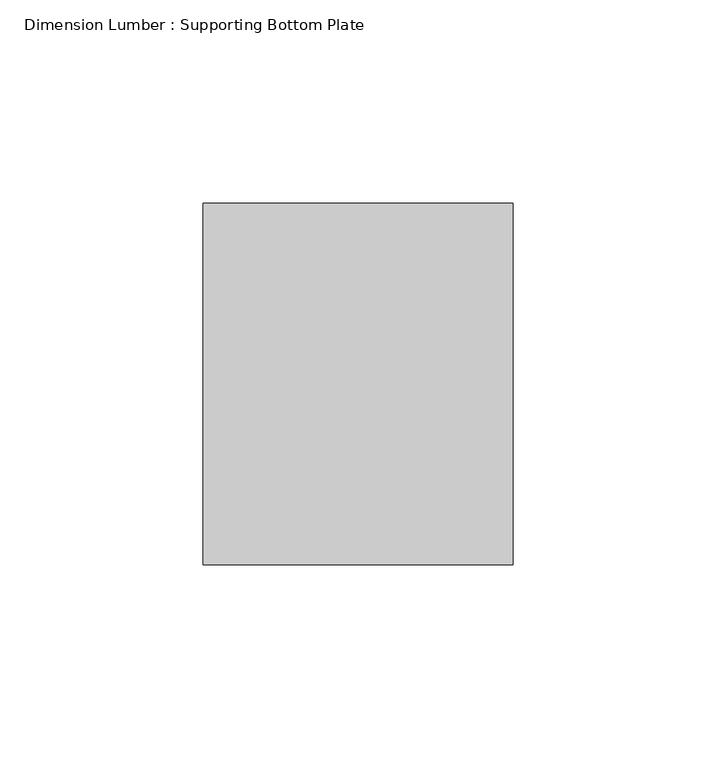
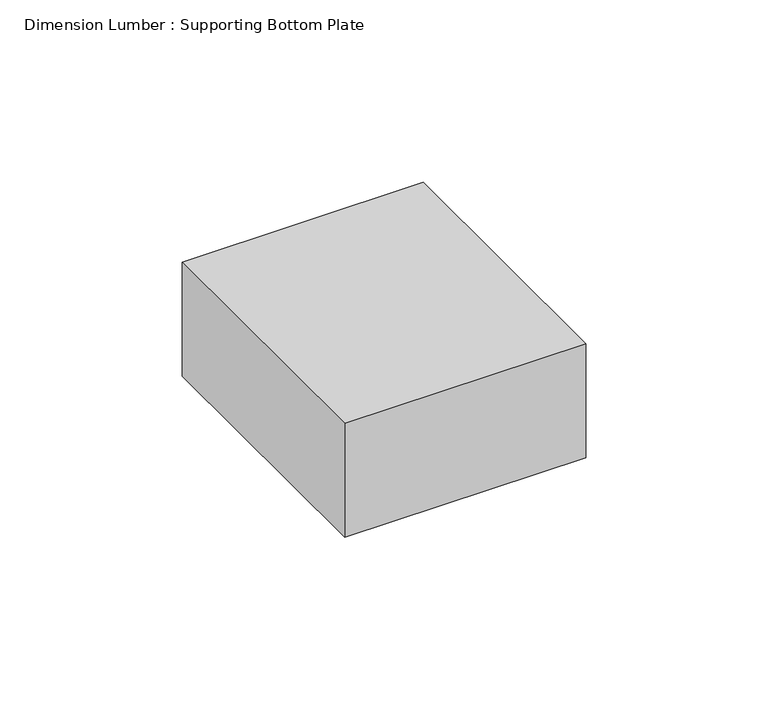
"""IFC4 building model written with IfcOpenShell, lengths in millimetres: beam geometry, Dimension Lumber : Supporting Bottom Plate."""

from ifc_helpers import new_model, si_unit, frame, origin, place, context, project, spatial, polyline, outline, extrude, source, transform, mapped, element, save


def dimension_lumber_supporting_bottom_plate_723ed126(model_context):
    return source(origin(), model_context, "Body", "SweptSolid", [
        extrude(outline(polyline([(60.325, 44.45), (60.325, -44.45), (-15.875, -44.45), (-15.875, 44.45), (60.325, 44.45)])), frame((0.0, 0.0, -19.05), z_axis=(0.0, 0.0, 1.0), x_axis=(1.0, 0.0, 0.0)), (0.0, 0.0, 1.0), 38.1),
    ])


if __name__ == "__main__":
    model = new_model("IFC4")
    model_context = context("Model", 3, world=origin())
    ifc_project = project(units=[si_unit("LENGTHUNIT", "METRE", prefix="MILLI")], contexts=[model_context])
    site = spatial("IfcSite", under=ifc_project)
    building = spatial("IfcBuilding", under=site)
    placement = place(None, origin())
    dimension_lumber_supporting_bottom_plate_shape = dimension_lumber_supporting_bottom_plate_723ed126(model_context)
    element("IfcBeam", 1, ObjectType="Dimension Lumber : Supporting Bottom Plate", at=placement, inside=building, context=model_context, shape_type="MappedRepresentation", body=[
        mapped(dimension_lumber_supporting_bottom_plate_shape, transform((0.0, 0.0, 0.0), x_axis=(1.0, 0.0, 0.0), y_axis=(0.0, 1.0, 0.0), z_axis=(0.0, 0.0, 1.0))),
    ])
    save(model, "model.ifc")

# Revit data of these elements
# Type "Dimension Lumber : Supporting Bottom Plate"
#   Assembly Code = "B10"
#   A = 0.0364583 SF
#   Length [instance default] = 5' - 0"
#   b = 0' - 3 1/2"
#   d = 0' - 1 1/2"
#   Structural Material [instance default] = Softwood, Lumber
# Element 1 (IfcBeam, "Dimension Lumber : Supporting Bottom Plate")
#   Structural Material = Douglas Fir #2
#   Materials on its faces: "Douglas Fir #2"
# Materials
#   "Softwood, Lumber": class "Wood", colour RGB 223 192 134, transparency 0, Description = "Pinus Echinata", Cost = 0
#   "Douglas Fir #2": class "Wood", colour RGB 223 192 134, transparency 0, Description = "Pinus Echinata", Cost = 0
